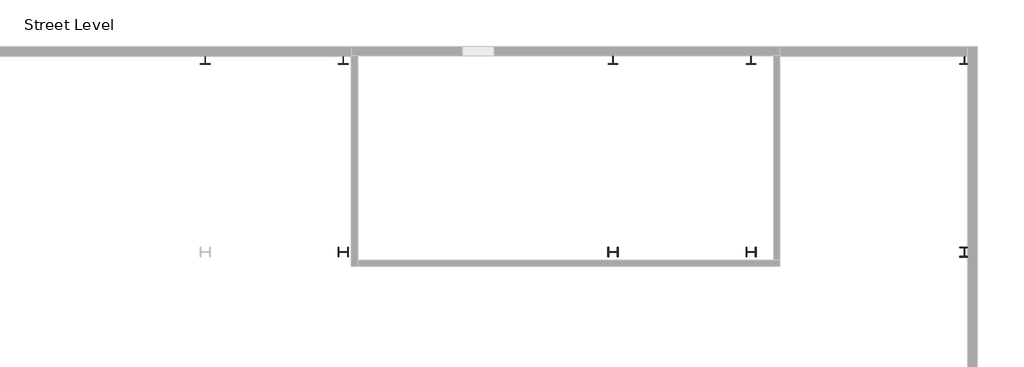
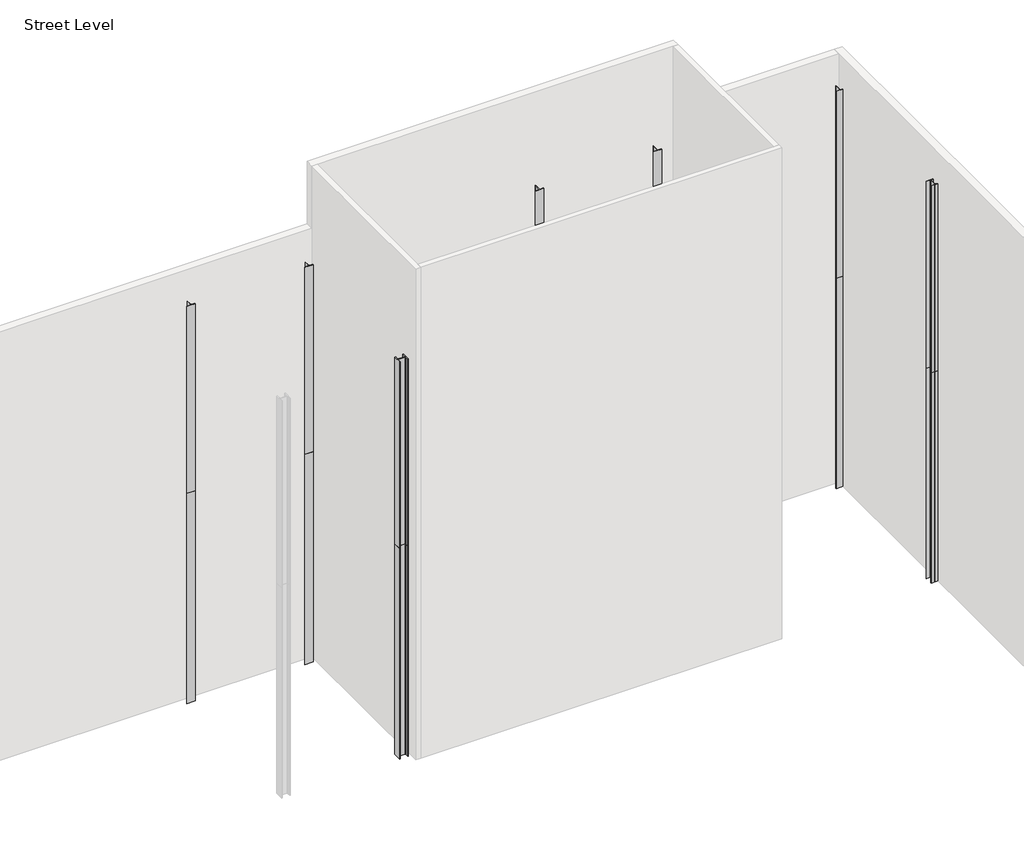
# One storey, part 3 of 3: 9 columns.
"""IFC4 building model written with IfcOpenShell, lengths in millimetres."""

from ifc_helpers import new_model, si_unit, point, frame, frame_2d, origin, place, context, project, spatial, polyline, circle_curve, trimmed, segment, composite_curve, outline, extrude, element, save

model = new_model("IFC4")

# Units and contexts
model_context = context("Model", 3, world=origin())
ifc_project = project(units=[si_unit("LENGTHUNIT", "METRE", prefix="MILLI")], contexts=[model_context])

# Site, building, storey
site = spatial("IfcSite", under=ifc_project)
building = spatial("IfcBuilding", under=site)
storey = spatial("IfcBuildingStorey", under=building, Name="Street Level", Elevation=-914.4)

# Columns
placement = place(None, origin())
element("IfcColumn", 1, ObjectType="W-Wide Flange-Column : W12X87", at=placement, inside=storey, context=model_context, shape_type="SweptSolid", body=[
    extrude(outline(composite_curve([segment(polyline([(-5274.2622732, 2940.2315304), (-5294.8362732, 2940.2315304), (-5294.8362732, 3065.0725304)]), True, "CONTINUOUS"), segment(trimmed(circle_curve(frame_2d((-5317.1247732, 3065.0725304)), 22.2885), [point((-5294.8362732, 3065.0725304))], [point((-5317.1247732, 3087.3610304))], True, "CARTESIAN"), True, "CONTINUOUS"), segment(polyline([(-5317.1247732, 3087.3610304), (-5548.8997732, 3087.3610304)]), True, "CONTINUOUS"), segment(trimmed(circle_curve(frame_2d((-5548.8997732, 3065.0725304)), 22.2885), [point((-5548.8997732, 3087.3610304))], [point((-5571.1882732, 3065.0725304))], True, "CARTESIAN"), True, "CONTINUOUS"), segment(polyline([(-5571.1882732, 3065.0725304), (-5571.1882732, 2940.2315304), (-5591.7622732, 2940.2315304), (-5591.7622732, 3247.5715304), (-5571.1882732, 3247.5715304), (-5571.1882732, 3122.7305304)]), True, "CONTINUOUS"), segment(trimmed(circle_curve(frame_2d((-5548.8997732, 3122.7305304)), 22.2885), [point((-5571.1882732, 3122.7305304))], [point((-5548.8997732, 3100.4420304))], True, "CARTESIAN"), True, "CONTINUOUS"), segment(polyline([(-5548.8997732, 3100.4420304), (-5317.1247732, 3100.4420304)]), True, "CONTINUOUS"), segment(trimmed(circle_curve(frame_2d((-5317.1247732, 3122.7305304)), 22.2885), [point((-5317.1247732, 3100.4420304))], [point((-5294.8362732, 3122.7305304))], True, "CARTESIAN"), True, "CONTINUOUS"), segment(polyline([(-5294.8362732, 3122.7305304), (-5294.8362732, 3247.5715304), (-5274.2622732, 3247.5715304), (-5274.2622732, 2940.2315304)]), True, "CONTINUOUS")], self_intersect=False)), frame((0.0, 0.0, 7315.2), z_axis=(0.0, 0.0, 1.0), x_axis=(1.0, 0.0, 0.0)), (0.0, 0.0, 1.0), 7315.2),
    extrude(outline(composite_curve([segment(polyline([(-5274.2622732, 2940.2315304), (-5294.8362732, 2940.2315304), (-5294.8362732, 3065.0725304)]), True, "CONTINUOUS"), segment(trimmed(circle_curve(frame_2d((-5317.1247732, 3065.0725304)), 22.2885), [point((-5294.8362732, 3065.0725304))], [point((-5317.1247732, 3087.3610304))], True, "CARTESIAN"), True, "CONTINUOUS"), segment(polyline([(-5317.1247732, 3087.3610304), (-5548.8997732, 3087.3610304)]), True, "CONTINUOUS"), segment(trimmed(circle_curve(frame_2d((-5548.8997732, 3065.0725304)), 22.2885), [point((-5548.8997732, 3087.3610304))], [point((-5571.1882732, 3065.0725304))], True, "CARTESIAN"), True, "CONTINUOUS"), segment(polyline([(-5571.1882732, 3065.0725304), (-5571.1882732, 2940.2315304), (-5591.7622732, 2940.2315304), (-5591.7622732, 3247.5715304), (-5571.1882732, 3247.5715304), (-5571.1882732, 3122.7305304)]), True, "CONTINUOUS"), segment(trimmed(circle_curve(frame_2d((-5548.8997732, 3122.7305304)), 22.2885), [point((-5571.1882732, 3122.7305304))], [point((-5548.8997732, 3100.4420304))], True, "CARTESIAN"), True, "CONTINUOUS"), segment(polyline([(-5548.8997732, 3100.4420304), (-5317.1247732, 3100.4420304)]), True, "CONTINUOUS"), segment(trimmed(circle_curve(frame_2d((-5317.1247732, 3122.7305304)), 22.2885), [point((-5317.1247732, 3100.4420304))], [point((-5294.8362732, 3122.7305304))], True, "CARTESIAN"), True, "CONTINUOUS"), segment(polyline([(-5294.8362732, 3122.7305304), (-5294.8362732, 3247.5715304), (-5274.2622732, 3247.5715304), (-5274.2622732, 2940.2315304)]), True, "CONTINUOUS")], self_intersect=False)), frame((0.0, 0.0, -914.4), z_axis=(0.0, 0.0, 1.0), x_axis=(1.0, 0.0, 0.0)), (0.0, 0.0, 1.0), 8229.6),
])
element("IfcColumn", 2, ObjectType="W-Wide Flange-Column : W12X87", at=placement, inside=storey, context=model_context, shape_type="SweptSolid", body=[
    extrude(outline(composite_curve([segment(polyline([(3260.1377268, 2940.2315304), (3239.5637268, 2940.2315304), (3239.5637268, 3065.0725304)]), True, "CONTINUOUS"), segment(trimmed(circle_curve(frame_2d((3217.2752268, 3065.0725304)), 22.2885), [point((3239.5637268, 3065.0725304))], [point((3217.2752268, 3087.3610304))], True, "CARTESIAN"), True, "CONTINUOUS"), segment(polyline([(3217.2752268, 3087.3610304), (2985.5002268, 3087.3610304)]), True, "CONTINUOUS"), segment(trimmed(circle_curve(frame_2d((2985.5002268, 3065.0725304)), 22.2885), [point((2985.5002268, 3087.3610304))], [point((2963.2117268, 3065.0725304))], True, "CARTESIAN"), True, "CONTINUOUS"), segment(polyline([(2963.2117268, 3065.0725304), (2963.2117268, 2940.2315304), (2942.6377268, 2940.2315304), (2942.6377268, 3247.5715304), (2963.2117268, 3247.5715304), (2963.2117268, 3122.7305304)]), True, "CONTINUOUS"), segment(trimmed(circle_curve(frame_2d((2985.5002268, 3122.7305304)), 22.2885), [point((2963.2117268, 3122.7305304))], [point((2985.5002268, 3100.4420304))], True, "CARTESIAN"), True, "CONTINUOUS"), segment(polyline([(2985.5002268, 3100.4420304), (3217.2752268, 3100.4420304)]), True, "CONTINUOUS"), segment(trimmed(circle_curve(frame_2d((3217.2752268, 3122.7305304)), 22.2885), [point((3217.2752268, 3100.4420304))], [point((3239.5637268, 3122.7305304))], True, "CARTESIAN"), True, "CONTINUOUS"), segment(polyline([(3239.5637268, 3122.7305304), (3239.5637268, 3247.5715304), (3260.1377268, 3247.5715304), (3260.1377268, 2940.2315304)]), True, "CONTINUOUS")], self_intersect=False)), frame((0.0, 0.0, 7315.2), z_axis=(0.0, 0.0, 1.0), x_axis=(1.0, 0.0, 0.0)), (0.0, 0.0, 1.0), 7315.2),
    extrude(outline(composite_curve([segment(polyline([(3260.1377268, 2940.2315304), (3239.5637268, 2940.2315304), (3239.5637268, 3065.0725304)]), True, "CONTINUOUS"), segment(trimmed(circle_curve(frame_2d((3217.2752268, 3065.0725304)), 22.2885), [point((3239.5637268, 3065.0725304))], [point((3217.2752268, 3087.3610304))], True, "CARTESIAN"), True, "CONTINUOUS"), segment(polyline([(3217.2752268, 3087.3610304), (2985.5002268, 3087.3610304)]), True, "CONTINUOUS"), segment(trimmed(circle_curve(frame_2d((2985.5002268, 3065.0725304)), 22.2885), [point((2985.5002268, 3087.3610304))], [point((2963.2117268, 3065.0725304))], True, "CARTESIAN"), True, "CONTINUOUS"), segment(polyline([(2963.2117268, 3065.0725304), (2963.2117268, 2940.2315304), (2942.6377268, 2940.2315304), (2942.6377268, 3247.5715304), (2963.2117268, 3247.5715304), (2963.2117268, 3122.7305304)]), True, "CONTINUOUS"), segment(trimmed(circle_curve(frame_2d((2985.5002268, 3122.7305304)), 22.2885), [point((2963.2117268, 3122.7305304))], [point((2985.5002268, 3100.4420304))], True, "CARTESIAN"), True, "CONTINUOUS"), segment(polyline([(2985.5002268, 3100.4420304), (3217.2752268, 3100.4420304)]), True, "CONTINUOUS"), segment(trimmed(circle_curve(frame_2d((3217.2752268, 3122.7305304)), 22.2885), [point((3217.2752268, 3100.4420304))], [point((3239.5637268, 3122.7305304))], True, "CARTESIAN"), True, "CONTINUOUS"), segment(polyline([(3239.5637268, 3122.7305304), (3239.5637268, 3247.5715304), (3260.1377268, 3247.5715304), (3260.1377268, 2940.2315304)]), True, "CONTINUOUS")], self_intersect=False)), frame((0.0, 0.0, -914.4), z_axis=(0.0, 0.0, 1.0), x_axis=(1.0, 0.0, 0.0)), (0.0, 0.0, 1.0), 8229.6),
])
element("IfcColumn", 3, ObjectType="W-Wide Flange-Column : W12X87", at=placement, inside=storey, context=model_context, shape_type="SweptSolid", body=[
    extrude(outline(composite_curve([segment(polyline([(7628.9377268, 2940.2315304), (7608.3637268, 2940.2315304), (7608.3637268, 3065.0725304)]), True, "CONTINUOUS"), segment(trimmed(circle_curve(frame_2d((7586.0752268, 3065.0725304)), 22.2885), [point((7608.3637268, 3065.0725304))], [point((7586.0752268, 3087.3610304))], True, "CARTESIAN"), True, "CONTINUOUS"), segment(polyline([(7586.0752268, 3087.3610304), (7354.3002268, 3087.3610304)]), True, "CONTINUOUS"), segment(trimmed(circle_curve(frame_2d((7354.3002268, 3065.0725304)), 22.2885), [point((7354.3002268, 3087.3610304))], [point((7332.0117268, 3065.0725304))], True, "CARTESIAN"), True, "CONTINUOUS"), segment(polyline([(7332.0117268, 3065.0725304), (7332.0117268, 2940.2315304), (7311.4377268, 2940.2315304), (7311.4377268, 3247.5715304), (7332.0117268, 3247.5715304), (7332.0117268, 3122.7305304)]), True, "CONTINUOUS"), segment(trimmed(circle_curve(frame_2d((7354.3002268, 3122.7305304)), 22.2885), [point((7332.0117268, 3122.7305304))], [point((7354.3002268, 3100.4420304))], True, "CARTESIAN"), True, "CONTINUOUS"), segment(polyline([(7354.3002268, 3100.4420304), (7586.0752268, 3100.4420304)]), True, "CONTINUOUS"), segment(trimmed(circle_curve(frame_2d((7586.0752268, 3122.7305304)), 22.2885), [point((7586.0752268, 3100.4420304))], [point((7608.3637268, 3122.7305304))], True, "CARTESIAN"), True, "CONTINUOUS"), segment(polyline([(7608.3637268, 3122.7305304), (7608.3637268, 3247.5715304), (7628.9377268, 3247.5715304), (7628.9377268, 2940.2315304)]), True, "CONTINUOUS")], self_intersect=False)), frame((0.0, 0.0, 7315.2), z_axis=(0.0, 0.0, 1.0), x_axis=(1.0, 0.0, 0.0)), (0.0, 0.0, 1.0), 7315.2),
    extrude(outline(composite_curve([segment(polyline([(7628.9377268, 2940.2315304), (7608.3637268, 2940.2315304), (7608.3637268, 3065.0725304)]), True, "CONTINUOUS"), segment(trimmed(circle_curve(frame_2d((7586.0752268, 3065.0725304)), 22.2885), [point((7608.3637268, 3065.0725304))], [point((7586.0752268, 3087.3610304))], True, "CARTESIAN"), True, "CONTINUOUS"), segment(polyline([(7586.0752268, 3087.3610304), (7354.3002268, 3087.3610304)]), True, "CONTINUOUS"), segment(trimmed(circle_curve(frame_2d((7354.3002268, 3065.0725304)), 22.2885), [point((7354.3002268, 3087.3610304))], [point((7332.0117268, 3065.0725304))], True, "CARTESIAN"), True, "CONTINUOUS"), segment(polyline([(7332.0117268, 3065.0725304), (7332.0117268, 2940.2315304), (7311.4377268, 2940.2315304), (7311.4377268, 3247.5715304), (7332.0117268, 3247.5715304), (7332.0117268, 3122.7305304)]), True, "CONTINUOUS"), segment(trimmed(circle_curve(frame_2d((7354.3002268, 3122.7305304)), 22.2885), [point((7332.0117268, 3122.7305304))], [point((7354.3002268, 3100.4420304))], True, "CARTESIAN"), True, "CONTINUOUS"), segment(polyline([(7354.3002268, 3100.4420304), (7586.0752268, 3100.4420304)]), True, "CONTINUOUS"), segment(trimmed(circle_curve(frame_2d((7586.0752268, 3122.7305304)), 22.2885), [point((7586.0752268, 3100.4420304))], [point((7608.3637268, 3122.7305304))], True, "CARTESIAN"), True, "CONTINUOUS"), segment(polyline([(7608.3637268, 3122.7305304), (7608.3637268, 3247.5715304), (7628.9377268, 3247.5715304), (7628.9377268, 2940.2315304)]), True, "CONTINUOUS")], self_intersect=False)), frame((0.0, 0.0, -914.4), z_axis=(0.0, 0.0, 1.0), x_axis=(1.0, 0.0, 0.0)), (0.0, 0.0, 1.0), 8229.6),
])
element("IfcColumn", 4, ObjectType="W-Wide Flange-Column : W12X87", at=placement, inside=storey, context=model_context, shape_type="SweptSolid", body=[
    extrude(outline(composite_curve([segment(polyline([(-9648.1422732, 9348.6515304), (-9648.1422732, 9328.0775304), (-9772.9832732, 9328.0775304)]), True, "CONTINUOUS"), segment(trimmed(circle_curve(frame_2d((-9772.9832732, 9305.7890304)), 22.2885), [point((-9772.9832732, 9328.0775304))], [point((-9795.2717732, 9305.7890304))], True, "CARTESIAN"), True, "CONTINUOUS"), segment(polyline([(-9795.2717732, 9305.7890304), (-9795.2717732, 9074.0140304)]), True, "CONTINUOUS"), segment(trimmed(circle_curve(frame_2d((-9772.9832732, 9074.0140304)), 22.2885), [point((-9795.2717732, 9074.0140304))], [point((-9772.9832732, 9051.7255304))], True, "CARTESIAN"), True, "CONTINUOUS"), segment(polyline([(-9772.9832732, 9051.7255304), (-9648.1422732, 9051.7255304), (-9648.1422732, 9031.1515304), (-9955.4822732, 9031.1515304), (-9955.4822732, 9051.7255304), (-9830.6412732, 9051.7255304)]), True, "CONTINUOUS"), segment(trimmed(circle_curve(frame_2d((-9830.6412732, 9074.0140304)), 22.2885), [point((-9830.6412732, 9051.7255304))], [point((-9808.3527732, 9074.0140304))], True, "CARTESIAN"), True, "CONTINUOUS"), segment(polyline([(-9808.3527732, 9074.0140304), (-9808.3527732, 9305.7890304)]), True, "CONTINUOUS"), segment(trimmed(circle_curve(frame_2d((-9830.6412732, 9305.7890304)), 22.2885), [point((-9808.3527732, 9305.7890304))], [point((-9830.6412732, 9328.0775304))], True, "CARTESIAN"), True, "CONTINUOUS"), segment(polyline([(-9830.6412732, 9328.0775304), (-9955.4822732, 9328.0775304), (-9955.4822732, 9348.6515304), (-9648.1422732, 9348.6515304)]), True, "CONTINUOUS")], self_intersect=False)), frame((0.0, 0.0, 7315.2), z_axis=(0.0, 0.0, 1.0), x_axis=(1.0, 0.0, 0.0)), (0.0, 0.0, 1.0), 7315.2),
    extrude(outline(composite_curve([segment(polyline([(-9648.1422732, 9348.6515304), (-9648.1422732, 9328.0775304), (-9772.9832732, 9328.0775304)]), True, "CONTINUOUS"), segment(trimmed(circle_curve(frame_2d((-9772.9832732, 9305.7890304)), 22.2885), [point((-9772.9832732, 9328.0775304))], [point((-9795.2717732, 9305.7890304))], True, "CARTESIAN"), True, "CONTINUOUS"), segment(polyline([(-9795.2717732, 9305.7890304), (-9795.2717732, 9074.0140304)]), True, "CONTINUOUS"), segment(trimmed(circle_curve(frame_2d((-9772.9832732, 9074.0140304)), 22.2885), [point((-9795.2717732, 9074.0140304))], [point((-9772.9832732, 9051.7255304))], True, "CARTESIAN"), True, "CONTINUOUS"), segment(polyline([(-9772.9832732, 9051.7255304), (-9648.1422732, 9051.7255304), (-9648.1422732, 9031.1515304), (-9955.4822732, 9031.1515304), (-9955.4822732, 9051.7255304), (-9830.6412732, 9051.7255304)]), True, "CONTINUOUS"), segment(trimmed(circle_curve(frame_2d((-9830.6412732, 9074.0140304)), 22.2885), [point((-9830.6412732, 9051.7255304))], [point((-9808.3527732, 9074.0140304))], True, "CARTESIAN"), True, "CONTINUOUS"), segment(polyline([(-9808.3527732, 9074.0140304), (-9808.3527732, 9305.7890304)]), True, "CONTINUOUS"), segment(trimmed(circle_curve(frame_2d((-9830.6412732, 9305.7890304)), 22.2885), [point((-9808.3527732, 9305.7890304))], [point((-9830.6412732, 9328.0775304))], True, "CARTESIAN"), True, "CONTINUOUS"), segment(polyline([(-9830.6412732, 9328.0775304), (-9955.4822732, 9328.0775304), (-9955.4822732, 9348.6515304), (-9648.1422732, 9348.6515304)]), True, "CONTINUOUS")], self_intersect=False)), frame((0.0, 0.0, -914.4), z_axis=(0.0, 0.0, 1.0), x_axis=(1.0, 0.0, 0.0)), (0.0, 0.0, 1.0), 8229.6),
])
element("IfcColumn", 5, ObjectType="W-Wide Flange-Column : W12X87", at=placement, inside=storey, context=model_context, shape_type="SweptSolid", body=[
    extrude(outline(composite_curve([segment(polyline([(-5279.3422732, 9348.6515304), (-5279.3422732, 9328.0775304), (-5404.1832732, 9328.0775304)]), True, "CONTINUOUS"), segment(trimmed(circle_curve(frame_2d((-5404.1832732, 9305.7890304)), 22.2885), [point((-5404.1832732, 9328.0775304))], [point((-5426.4717732, 9305.7890304))], True, "CARTESIAN"), True, "CONTINUOUS"), segment(polyline([(-5426.4717732, 9305.7890304), (-5426.4717732, 9074.0140304)]), True, "CONTINUOUS"), segment(trimmed(circle_curve(frame_2d((-5404.1832732, 9074.0140304)), 22.2885), [point((-5426.4717732, 9074.0140304))], [point((-5404.1832732, 9051.7255304))], True, "CARTESIAN"), True, "CONTINUOUS"), segment(polyline([(-5404.1832732, 9051.7255304), (-5279.3422732, 9051.7255304), (-5279.3422732, 9031.1515304), (-5586.6822732, 9031.1515304), (-5586.6822732, 9051.7255304), (-5461.8412732, 9051.7255304)]), True, "CONTINUOUS"), segment(trimmed(circle_curve(frame_2d((-5461.8412732, 9074.0140304)), 22.2885), [point((-5461.8412732, 9051.7255304))], [point((-5439.5527732, 9074.0140304))], True, "CARTESIAN"), True, "CONTINUOUS"), segment(polyline([(-5439.5527732, 9074.0140304), (-5439.5527732, 9305.7890304)]), True, "CONTINUOUS"), segment(trimmed(circle_curve(frame_2d((-5461.8412732, 9305.7890304)), 22.2885), [point((-5439.5527732, 9305.7890304))], [point((-5461.8412732, 9328.0775304))], True, "CARTESIAN"), True, "CONTINUOUS"), segment(polyline([(-5461.8412732, 9328.0775304), (-5586.6822732, 9328.0775304), (-5586.6822732, 9348.6515304), (-5279.3422732, 9348.6515304)]), True, "CONTINUOUS")], self_intersect=False)), frame((0.0, 0.0, 7315.2), z_axis=(0.0, 0.0, 1.0), x_axis=(1.0, 0.0, 0.0)), (0.0, 0.0, 1.0), 7315.2),
    extrude(outline(composite_curve([segment(polyline([(-5279.3422732, 9348.6515304), (-5279.3422732, 9328.0775304), (-5404.1832732, 9328.0775304)]), True, "CONTINUOUS"), segment(trimmed(circle_curve(frame_2d((-5404.1832732, 9305.7890304)), 22.2885), [point((-5404.1832732, 9328.0775304))], [point((-5426.4717732, 9305.7890304))], True, "CARTESIAN"), True, "CONTINUOUS"), segment(polyline([(-5426.4717732, 9305.7890304), (-5426.4717732, 9074.0140304)]), True, "CONTINUOUS"), segment(trimmed(circle_curve(frame_2d((-5404.1832732, 9074.0140304)), 22.2885), [point((-5426.4717732, 9074.0140304))], [point((-5404.1832732, 9051.7255304))], True, "CARTESIAN"), True, "CONTINUOUS"), segment(polyline([(-5404.1832732, 9051.7255304), (-5279.3422732, 9051.7255304), (-5279.3422732, 9031.1515304), (-5586.6822732, 9031.1515304), (-5586.6822732, 9051.7255304), (-5461.8412732, 9051.7255304)]), True, "CONTINUOUS"), segment(trimmed(circle_curve(frame_2d((-5461.8412732, 9074.0140304)), 22.2885), [point((-5461.8412732, 9051.7255304))], [point((-5439.5527732, 9074.0140304))], True, "CARTESIAN"), True, "CONTINUOUS"), segment(polyline([(-5439.5527732, 9074.0140304), (-5439.5527732, 9305.7890304)]), True, "CONTINUOUS"), segment(trimmed(circle_curve(frame_2d((-5461.8412732, 9305.7890304)), 22.2885), [point((-5439.5527732, 9305.7890304))], [point((-5461.8412732, 9328.0775304))], True, "CARTESIAN"), True, "CONTINUOUS"), segment(polyline([(-5461.8412732, 9328.0775304), (-5586.6822732, 9328.0775304), (-5586.6822732, 9348.6515304), (-5279.3422732, 9348.6515304)]), True, "CONTINUOUS")], self_intersect=False)), frame((0.0, 0.0, -914.4), z_axis=(0.0, 0.0, 1.0), x_axis=(1.0, 0.0, 0.0)), (0.0, 0.0, 1.0), 8229.6),
])
element("IfcColumn", 6, ObjectType="W-Wide Flange-Column : W12X87", at=placement, inside=storey, context=model_context, shape_type="SweptSolid", body=[
    extrude(outline(composite_curve([segment(polyline([(3255.0577268, 9348.6515304), (3255.0577268, 9328.0775304), (3130.2167268, 9328.0775304)]), True, "CONTINUOUS"), segment(trimmed(circle_curve(frame_2d((3130.2167268, 9305.7890304)), 22.2885), [point((3130.2167268, 9328.0775304))], [point((3107.9282268, 9305.7890304))], True, "CARTESIAN"), True, "CONTINUOUS"), segment(polyline([(3107.9282268, 9305.7890304), (3107.9282268, 9074.0140304)]), True, "CONTINUOUS"), segment(trimmed(circle_curve(frame_2d((3130.2167268, 9074.0140304)), 22.2885), [point((3107.9282268, 9074.0140304))], [point((3130.2167268, 9051.7255304))], True, "CARTESIAN"), True, "CONTINUOUS"), segment(polyline([(3130.2167268, 9051.7255304), (3255.0577268, 9051.7255304), (3255.0577268, 9031.1515304), (2947.7177268, 9031.1515304), (2947.7177268, 9051.7255304), (3072.5587268, 9051.7255304)]), True, "CONTINUOUS"), segment(trimmed(circle_curve(frame_2d((3072.5587268, 9074.0140304)), 22.2885), [point((3072.5587268, 9051.7255304))], [point((3094.8472268, 9074.0140304))], True, "CARTESIAN"), True, "CONTINUOUS"), segment(polyline([(3094.8472268, 9074.0140304), (3094.8472268, 9305.7890304)]), True, "CONTINUOUS"), segment(trimmed(circle_curve(frame_2d((3072.5587268, 9305.7890304)), 22.2885), [point((3094.8472268, 9305.7890304))], [point((3072.5587268, 9328.0775304))], True, "CARTESIAN"), True, "CONTINUOUS"), segment(polyline([(3072.5587268, 9328.0775304), (2947.7177268, 9328.0775304), (2947.7177268, 9348.6515304), (3255.0577268, 9348.6515304)]), True, "CONTINUOUS")], self_intersect=False)), frame((0.0, 0.0, 7315.2), z_axis=(0.0, 0.0, 1.0), x_axis=(1.0, 0.0, 0.0)), (0.0, 0.0, 1.0), 7315.2),
    extrude(outline(composite_curve([segment(polyline([(3255.0577268, 9348.6515304), (3255.0577268, 9328.0775304), (3130.2167268, 9328.0775304)]), True, "CONTINUOUS"), segment(trimmed(circle_curve(frame_2d((3130.2167268, 9305.7890304)), 22.2885), [point((3130.2167268, 9328.0775304))], [point((3107.9282268, 9305.7890304))], True, "CARTESIAN"), True, "CONTINUOUS"), segment(polyline([(3107.9282268, 9305.7890304), (3107.9282268, 9074.0140304)]), True, "CONTINUOUS"), segment(trimmed(circle_curve(frame_2d((3130.2167268, 9074.0140304)), 22.2885), [point((3107.9282268, 9074.0140304))], [point((3130.2167268, 9051.7255304))], True, "CARTESIAN"), True, "CONTINUOUS"), segment(polyline([(3130.2167268, 9051.7255304), (3255.0577268, 9051.7255304), (3255.0577268, 9031.1515304), (2947.7177268, 9031.1515304), (2947.7177268, 9051.7255304), (3072.5587268, 9051.7255304)]), True, "CONTINUOUS"), segment(trimmed(circle_curve(frame_2d((3072.5587268, 9074.0140304)), 22.2885), [point((3072.5587268, 9051.7255304))], [point((3094.8472268, 9074.0140304))], True, "CARTESIAN"), True, "CONTINUOUS"), segment(polyline([(3094.8472268, 9074.0140304), (3094.8472268, 9305.7890304)]), True, "CONTINUOUS"), segment(trimmed(circle_curve(frame_2d((3072.5587268, 9305.7890304)), 22.2885), [point((3094.8472268, 9305.7890304))], [point((3072.5587268, 9328.0775304))], True, "CARTESIAN"), True, "CONTINUOUS"), segment(polyline([(3072.5587268, 9328.0775304), (2947.7177268, 9328.0775304), (2947.7177268, 9348.6515304), (3255.0577268, 9348.6515304)]), True, "CONTINUOUS")], self_intersect=False)), frame((0.0, 0.0, -914.4), z_axis=(0.0, 0.0, 1.0), x_axis=(1.0, 0.0, 0.0)), (0.0, 0.0, 1.0), 8229.6),
])
element("IfcColumn", 7, ObjectType="W-Wide Flange-Column : W12X87", at=placement, inside=storey, context=model_context, shape_type="SweptSolid", body=[
    extrude(outline(composite_curve([segment(polyline([(7623.8577268, 9348.6515304), (7623.8577268, 9328.0775304), (7499.0167268, 9328.0775304)]), True, "CONTINUOUS"), segment(trimmed(circle_curve(frame_2d((7499.0167268, 9305.7890304)), 22.2885), [point((7499.0167268, 9328.0775304))], [point((7476.7282268, 9305.7890304))], True, "CARTESIAN"), True, "CONTINUOUS"), segment(polyline([(7476.7282268, 9305.7890304), (7476.7282268, 9074.0140304)]), True, "CONTINUOUS"), segment(trimmed(circle_curve(frame_2d((7499.0167268, 9074.0140304)), 22.2885), [point((7476.7282268, 9074.0140304))], [point((7499.0167268, 9051.7255304))], True, "CARTESIAN"), True, "CONTINUOUS"), segment(polyline([(7499.0167268, 9051.7255304), (7623.8577268, 9051.7255304), (7623.8577268, 9031.1515304), (7316.5177268, 9031.1515304), (7316.5177268, 9051.7255304), (7441.3587268, 9051.7255304)]), True, "CONTINUOUS"), segment(trimmed(circle_curve(frame_2d((7441.3587268, 9074.0140304)), 22.2885), [point((7441.3587268, 9051.7255304))], [point((7463.6472268, 9074.0140304))], True, "CARTESIAN"), True, "CONTINUOUS"), segment(polyline([(7463.6472268, 9074.0140304), (7463.6472268, 9305.7890304)]), True, "CONTINUOUS"), segment(trimmed(circle_curve(frame_2d((7441.3587268, 9305.7890304)), 22.2885), [point((7463.6472268, 9305.7890304))], [point((7441.3587268, 9328.0775304))], True, "CARTESIAN"), True, "CONTINUOUS"), segment(polyline([(7441.3587268, 9328.0775304), (7316.5177268, 9328.0775304), (7316.5177268, 9348.6515304), (7623.8577268, 9348.6515304)]), True, "CONTINUOUS")], self_intersect=False)), frame((0.0, 0.0, 7315.2), z_axis=(0.0, 0.0, 1.0), x_axis=(1.0, 0.0, 0.0)), (0.0, 0.0, 1.0), 7315.2),
    extrude(outline(composite_curve([segment(polyline([(7623.8577268, 9348.6515304), (7623.8577268, 9328.0775304), (7499.0167268, 9328.0775304)]), True, "CONTINUOUS"), segment(trimmed(circle_curve(frame_2d((7499.0167268, 9305.7890304)), 22.2885), [point((7499.0167268, 9328.0775304))], [point((7476.7282268, 9305.7890304))], True, "CARTESIAN"), True, "CONTINUOUS"), segment(polyline([(7476.7282268, 9305.7890304), (7476.7282268, 9074.0140304)]), True, "CONTINUOUS"), segment(trimmed(circle_curve(frame_2d((7499.0167268, 9074.0140304)), 22.2885), [point((7476.7282268, 9074.0140304))], [point((7499.0167268, 9051.7255304))], True, "CARTESIAN"), True, "CONTINUOUS"), segment(polyline([(7499.0167268, 9051.7255304), (7623.8577268, 9051.7255304), (7623.8577268, 9031.1515304), (7316.5177268, 9031.1515304), (7316.5177268, 9051.7255304), (7441.3587268, 9051.7255304)]), True, "CONTINUOUS"), segment(trimmed(circle_curve(frame_2d((7441.3587268, 9074.0140304)), 22.2885), [point((7441.3587268, 9051.7255304))], [point((7463.6472268, 9074.0140304))], True, "CARTESIAN"), True, "CONTINUOUS"), segment(polyline([(7463.6472268, 9074.0140304), (7463.6472268, 9305.7890304)]), True, "CONTINUOUS"), segment(trimmed(circle_curve(frame_2d((7441.3587268, 9305.7890304)), 22.2885), [point((7463.6472268, 9305.7890304))], [point((7441.3587268, 9328.0775304))], True, "CARTESIAN"), True, "CONTINUOUS"), segment(polyline([(7441.3587268, 9328.0775304), (7316.5177268, 9328.0775304), (7316.5177268, 9348.6515304), (7623.8577268, 9348.6515304)]), True, "CONTINUOUS")], self_intersect=False)), frame((0.0, 0.0, -914.4), z_axis=(0.0, 0.0, 1.0), x_axis=(1.0, 0.0, 0.0)), (0.0, 0.0, 1.0), 8229.6),
])
element("IfcColumn", 8, ObjectType="W-Wide Flange-Column : W12X87", at=placement, inside=storey, context=model_context, shape_type="SweptSolid", body=[
    extrude(outline(composite_curve([segment(polyline([(14380.2577268, 9348.6515304), (14380.2577268, 9328.0775304), (14255.4167268, 9328.0775304)]), True, "CONTINUOUS"), segment(trimmed(circle_curve(frame_2d((14255.4167268, 9305.7890304)), 22.2885), [point((14255.4167268, 9328.0775304))], [point((14233.1282268, 9305.7890304))], True, "CARTESIAN"), True, "CONTINUOUS"), segment(polyline([(14233.1282268, 9305.7890304), (14233.1282268, 9074.0140304)]), True, "CONTINUOUS"), segment(trimmed(circle_curve(frame_2d((14255.4167268, 9074.0140304)), 22.2885), [point((14233.1282268, 9074.0140304))], [point((14255.4167268, 9051.7255304))], True, "CARTESIAN"), True, "CONTINUOUS"), segment(polyline([(14255.4167268, 9051.7255304), (14380.2577268, 9051.7255304), (14380.2577268, 9031.1515304), (14072.9177268, 9031.1515304), (14072.9177268, 9051.7255304), (14197.7587268, 9051.7255304)]), True, "CONTINUOUS"), segment(trimmed(circle_curve(frame_2d((14197.7587268, 9074.0140304)), 22.2885), [point((14197.7587268, 9051.7255304))], [point((14220.0472268, 9074.0140304))], True, "CARTESIAN"), True, "CONTINUOUS"), segment(polyline([(14220.0472268, 9074.0140304), (14220.0472268, 9305.7890304)]), True, "CONTINUOUS"), segment(trimmed(circle_curve(frame_2d((14197.7587268, 9305.7890304)), 22.2885), [point((14220.0472268, 9305.7890304))], [point((14197.7587268, 9328.0775304))], True, "CARTESIAN"), True, "CONTINUOUS"), segment(polyline([(14197.7587268, 9328.0775304), (14072.9177268, 9328.0775304), (14072.9177268, 9348.6515304), (14380.2577268, 9348.6515304)]), True, "CONTINUOUS")], self_intersect=False)), frame((0.0, 0.0, 7315.2), z_axis=(0.0, 0.0, 1.0), x_axis=(1.0, 0.0, 0.0)), (0.0, 0.0, 1.0), 7315.2),
    extrude(outline(composite_curve([segment(polyline([(14380.2577268, 9348.6515304), (14380.2577268, 9328.0775304), (14255.4167268, 9328.0775304)]), True, "CONTINUOUS"), segment(trimmed(circle_curve(frame_2d((14255.4167268, 9305.7890304)), 22.2885), [point((14255.4167268, 9328.0775304))], [point((14233.1282268, 9305.7890304))], True, "CARTESIAN"), True, "CONTINUOUS"), segment(polyline([(14233.1282268, 9305.7890304), (14233.1282268, 9074.0140304)]), True, "CONTINUOUS"), segment(trimmed(circle_curve(frame_2d((14255.4167268, 9074.0140304)), 22.2885), [point((14233.1282268, 9074.0140304))], [point((14255.4167268, 9051.7255304))], True, "CARTESIAN"), True, "CONTINUOUS"), segment(polyline([(14255.4167268, 9051.7255304), (14380.2577268, 9051.7255304), (14380.2577268, 9031.1515304), (14072.9177268, 9031.1515304), (14072.9177268, 9051.7255304), (14197.7587268, 9051.7255304)]), True, "CONTINUOUS"), segment(trimmed(circle_curve(frame_2d((14197.7587268, 9074.0140304)), 22.2885), [point((14197.7587268, 9051.7255304))], [point((14220.0472268, 9074.0140304))], True, "CARTESIAN"), True, "CONTINUOUS"), segment(polyline([(14220.0472268, 9074.0140304), (14220.0472268, 9305.7890304)]), True, "CONTINUOUS"), segment(trimmed(circle_curve(frame_2d((14197.7587268, 9305.7890304)), 22.2885), [point((14220.0472268, 9305.7890304))], [point((14197.7587268, 9328.0775304))], True, "CARTESIAN"), True, "CONTINUOUS"), segment(polyline([(14197.7587268, 9328.0775304), (14072.9177268, 9328.0775304), (14072.9177268, 9348.6515304), (14380.2577268, 9348.6515304)]), True, "CONTINUOUS")], self_intersect=False)), frame((0.0, 0.0, -914.4), z_axis=(0.0, 0.0, 1.0), x_axis=(1.0, 0.0, 0.0)), (0.0, 0.0, 1.0), 8229.6),
])
element("IfcColumn", 9, ObjectType="W-Wide Flange-Column : W12X87", at=placement, inside=storey, context=model_context, shape_type="SweptSolid", body=[
    extrude(outline(composite_curve([segment(polyline([(14380.2577268, 3252.6515304), (14380.2577268, 3232.0775304), (14255.4167268, 3232.0775304)]), True, "CONTINUOUS"), segment(trimmed(circle_curve(frame_2d((14255.4167268, 3209.7890304)), 22.2885), [point((14255.4167268, 3232.0775304))], [point((14233.1282268, 3209.7890304))], True, "CARTESIAN"), True, "CONTINUOUS"), segment(polyline([(14233.1282268, 3209.7890304), (14233.1282268, 2978.0140304)]), True, "CONTINUOUS"), segment(trimmed(circle_curve(frame_2d((14255.4167268, 2978.0140304)), 22.2885), [point((14233.1282268, 2978.0140304))], [point((14255.4167268, 2955.7255304))], True, "CARTESIAN"), True, "CONTINUOUS"), segment(polyline([(14255.4167268, 2955.7255304), (14380.2577268, 2955.7255304), (14380.2577268, 2935.1515304), (14072.9177268, 2935.1515304), (14072.9177268, 2955.7255304), (14197.7587268, 2955.7255304)]), True, "CONTINUOUS"), segment(trimmed(circle_curve(frame_2d((14197.7587268, 2978.0140304)), 22.2885), [point((14197.7587268, 2955.7255304))], [point((14220.0472268, 2978.0140304))], True, "CARTESIAN"), True, "CONTINUOUS"), segment(polyline([(14220.0472268, 2978.0140304), (14220.0472268, 3209.7890304)]), True, "CONTINUOUS"), segment(trimmed(circle_curve(frame_2d((14197.7587268, 3209.7890304)), 22.2885), [point((14220.0472268, 3209.7890304))], [point((14197.7587268, 3232.0775304))], True, "CARTESIAN"), True, "CONTINUOUS"), segment(polyline([(14197.7587268, 3232.0775304), (14072.9177268, 3232.0775304), (14072.9177268, 3252.6515304), (14380.2577268, 3252.6515304)]), True, "CONTINUOUS")], self_intersect=False)), frame((0.0, 0.0, 7315.2), z_axis=(0.0, 0.0, 1.0), x_axis=(1.0, 0.0, 0.0)), (0.0, 0.0, 1.0), 7315.2),
    extrude(outline(composite_curve([segment(polyline([(14380.2577268, 3252.6515304), (14380.2577268, 3232.0775304), (14255.4167268, 3232.0775304)]), True, "CONTINUOUS"), segment(trimmed(circle_curve(frame_2d((14255.4167268, 3209.7890304)), 22.2885), [point((14255.4167268, 3232.0775304))], [point((14233.1282268, 3209.7890304))], True, "CARTESIAN"), True, "CONTINUOUS"), segment(polyline([(14233.1282268, 3209.7890304), (14233.1282268, 2978.0140304)]), True, "CONTINUOUS"), segment(trimmed(circle_curve(frame_2d((14255.4167268, 2978.0140304)), 22.2885), [point((14233.1282268, 2978.0140304))], [point((14255.4167268, 2955.7255304))], True, "CARTESIAN"), True, "CONTINUOUS"), segment(polyline([(14255.4167268, 2955.7255304), (14380.2577268, 2955.7255304), (14380.2577268, 2935.1515304), (14072.9177268, 2935.1515304), (14072.9177268, 2955.7255304), (14197.7587268, 2955.7255304)]), True, "CONTINUOUS"), segment(trimmed(circle_curve(frame_2d((14197.7587268, 2978.0140304)), 22.2885), [point((14197.7587268, 2955.7255304))], [point((14220.0472268, 2978.0140304))], True, "CARTESIAN"), True, "CONTINUOUS"), segment(polyline([(14220.0472268, 2978.0140304), (14220.0472268, 3209.7890304)]), True, "CONTINUOUS"), segment(trimmed(circle_curve(frame_2d((14197.7587268, 3209.7890304)), 22.2885), [point((14220.0472268, 3209.7890304))], [point((14197.7587268, 3232.0775304))], True, "CARTESIAN"), True, "CONTINUOUS"), segment(polyline([(14197.7587268, 3232.0775304), (14072.9177268, 3232.0775304), (14072.9177268, 3252.6515304), (14380.2577268, 3252.6515304)]), True, "CONTINUOUS")], self_intersect=False)), frame((0.0, 0.0, -914.4), z_axis=(0.0, 0.0, 1.0), x_axis=(1.0, 0.0, 0.0)), (0.0, 0.0, 1.0), 8229.6),
])

save(model, "model.ifc")

# Revit data of these elements
# Project information
#   Organization Name = "G3B Press"
#   Organization Description = "Paul F. Aubin Cosulting Services, Inc."
#   Building Name = "Revit Essentials for Architecture"
#   Author = "Paul F. Aubin"
#   Author Website = "https://www.paulaubin.com"
#   Copyright = "Copyright © 2020 Paul F Aubin, all rights reserved"
#   Project Issue Date = "8/1/2020"
#   Project Status = "Design Development"
#   Client Name = "Groups and Links"
#   Project Address = "123 State ST\nSuite 301\nChicago, IL 60606"
#   Project Name = "07 Commercial_Complete"
#   Project Number = "2020.04A"
# Grids (mm)
#   "1": line (-22547.601, -9504.498) -> (19277.595, -9504.498)
#   "2": line (-22547.601, -3408.498) -> (19277.595, -3408.498)
#   "3": line (-22547.601, 3093.902) -> (19277.595, 3093.902)
#   "4": line (-22547.601, 9189.902) -> (19277.595, 9189.902)
#   "A": line (-16558.212, 12259.726) -> (-16558.212, -14197.104)
#   "B": line (-9801.812, 12259.726) -> (-9801.812, -14197.104)
#   "C": line (-5433.012, 12259.726) -> (-5433.012, -14197.104)
#   "D": line (3101.388, 12259.726) -> (3101.388, -14197.104)
#   "E": line (7470.188, 12259.726) -> (7470.188, -14197.104)
#   "F": line (14226.588, 12259.726) -> (14226.588, -14197.104)
#   "C.3": line (-2689.812, -15151.11) -> (-2689.812, -5965.346)
#   "C.7": line (358.188, -15151.11) -> (358.188, -5965.346)
# Type "W-Wide Flange-Column : W12X87"
#   Assembly Code = "B10"
#   W = 87
#   bf = 1' - 0.1"
#   d = 1' - 0 1/2"
#   k = 0' - 1 11/16"
#   kr = 0' - 0.8775"
#   tf = 0' - 0.81"
#   tw = 0' - 0.515"
#   A = 0.177778 SF
#   Structural Material [instance default] = Steel ASTM A992
# Elements 1, 2, 3, 4, 5, 6, 7, 8, 9 (IfcColumn, "W-Wide Flange-Column : W12X87")
#   Structural Material = Steel ASTM A992
#   Phase Created = New Construction
#   Materials on its faces: "Steel ASTM A992"
# Materials
#   "Steel ASTM A992": class "Metal", colour RGB 199 199 199, transparency 0, Description = "Structural steel 50ksi", Cost = 0
